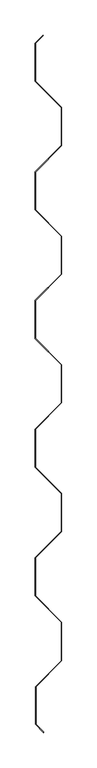
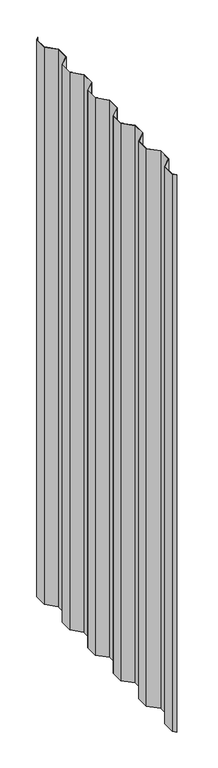
"""IFC4 building model written with IfcOpenShell, lengths in millimetres: proxy geometry, MBCI 7.2-V Panel15 : MBCI 7.2-V Panel-1."""

from ifc_helpers import new_model, si_unit, frame, origin, place, context, project, spatial, polyline, outline, extrude, source, transform, mapped, element, save


def generic_models_ff516ca3(model_context):
    return source(origin(), model_context, "Body", "SweptSolid", [
        extrude(outline(polyline([(590353.5827614, -532525.5919067), (590353.5827614, -532471.4801976), (590364.9833956, -532460.0795634), (590365.0253204, -532460.8795376), (590354.1780739, -532471.7267841), (590354.1780739, -532525.3453202), (590391.6684739, -532562.8357202), (590391.6684739, -532617.1163841), (590354.1780739, -532654.6067841), (590354.1780739, -532708.2253202), (590391.6684739, -532745.7157202), (590391.6684739, -532799.9963841), (590354.1780739, -532837.4867841), (590354.1780739, -532891.1053202), (590391.6684739, -532928.5957202), (590391.6684739, -532982.8763841), (590354.1780739, -533020.3667841), (590354.1780739, -533073.9853202), (590391.6684739, -533111.4757202), (590391.6684739, -533165.7563841), (590354.1780739, -533203.2467841), (590354.1780739, -533256.8653202), (590391.6684739, -533294.3557202), (590391.6684739, -533349.4999841), (590354.7876739, -533386.3807841), (590354.7876739, -533439.4689111), (590365.9181078, -533450.599345), (590365.8630841, -533451.3862203), (590354.1923614, -533439.7154976), (590354.1923614, -533386.1341976), (590391.0731614, -533349.2533976), (590391.0731614, -533294.6023067), (590353.5827614, -533257.1119067), (590353.5827614, -533203.0001976), (590391.0731614, -533165.5097976), (590391.0731614, -533111.7223067), (590353.5827614, -533074.2319067), (590353.5827614, -533020.1201976), (590391.0731614, -532982.6297976), (590391.0731614, -532928.8423067), (590353.5827614, -532891.3519067), (590353.5827614, -532837.2401976), (590391.0731614, -532799.7497976), (590391.0731614, -532745.9623067), (590353.5827614, -532708.4719067), (590353.5827614, -532654.3601976), (590391.0731614, -532616.8697976), (590391.0731614, -532563.0823067), (590353.5827614, -532525.5919067)])), frame((0.0, 0.0, 6.35), z_axis=(0.0, 0.0, 1.0), x_axis=(1.0, 0.0, 0.0)), (0.0, 0.0, 1.0), 2432.05),
    ])


if __name__ == "__main__":
    model = new_model("IFC4")
    model_context = context("Model", 3, world=origin())
    ifc_project = project(units=[si_unit("LENGTHUNIT", "METRE", prefix="MILLI")], contexts=[model_context])
    site = spatial("IfcSite", under=ifc_project)
    building = spatial("IfcBuilding", under=site)
    placement = place(None, origin())
    generic_models_shape = generic_models_ff516ca3(model_context)
    element("IfcBuildingElementProxy", 1, Name="MBCI 7.2-V Panel15 : MBCI 7.2-V Panel-1", ObjectType="MBCI 7.2-V Panel15 : MBCI 7.2-V Panel-1", at=placement, inside=building, context=model_context, shape_type="MappedRepresentation", body=[
        mapped(generic_models_shape, transform((0.0, 0.0, 0.0), x_axis=(1.0, 0.0, 0.0), y_axis=(0.0, 1.0, 0.0), z_axis=(0.0, 0.0, 1.0))),
    ])
    save(model, "model.ifc")

# Revit data of these elements
# Element 1 (IfcBuildingElementProxy, "MBCI 7.2-V Panel15 : MBCI 7.2-V Panel-1")
#   Materials on its faces: "MTL PANEL"
# Materials
#   "MTL PANEL": class "Generic", colour RGB 239 242 240, transparency 0, Cost = 0
